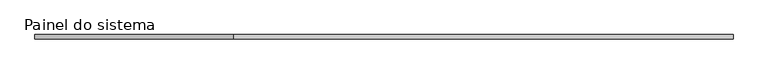
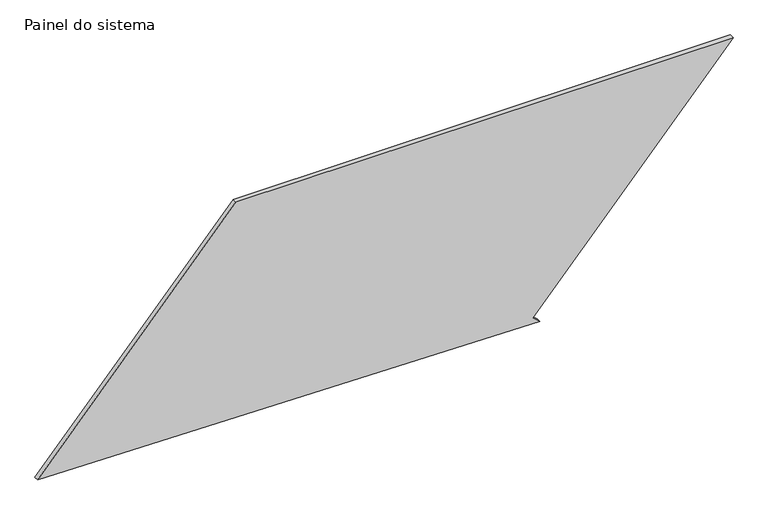
"""IFC4 building model written with IfcOpenShell, lengths in millimetres: plate geometry, Painel do sistema : Envidraçado."""

from ifc_helpers import new_model, si_unit, frame, origin, place, context, project, spatial, polyline, outline, extrude, source, transform, mapped, element, save


def painel_do_sistema_1ee32824(model_context):
    return source(origin(), model_context, "Body", "SweptSolid", [
        extrude(outline(polyline([(0.0, 853.2973256), (33.0713273, 815.7968281), (1287.5514622, 1922.1107677), (1287.5514622, -826.9931544), (45.767153, -1922.1107677), (0.0, 853.2973256)])), frame((0.0, 24.5, 0.0), z_axis=(0.0, 1.0, 0.0), x_axis=(0.0, 0.0, 1.0)), (0.0, 0.0, 1.0), 25.0),
    ])


if __name__ == "__main__":
    model = new_model("IFC4")
    model_context = context("Model", 3, world=origin())
    ifc_project = project(units=[si_unit("LENGTHUNIT", "METRE", prefix="MILLI")], contexts=[model_context])
    site = spatial("IfcSite", under=ifc_project)
    building = spatial("IfcBuilding", under=site)
    placement = place(None, origin())
    painel_do_sistema_shape = painel_do_sistema_1ee32824(model_context)
    element("IfcPlate", 1, ObjectType="Painel do sistema : Envidraçado", at=placement, inside=building, context=model_context, shape_type="MappedRepresentation", body=[
        mapped(painel_do_sistema_shape, transform((0.0, 0.0, 0.0), x_axis=(1.0, 0.0, 0.0), y_axis=(0.0, 1.0, 0.0), z_axis=(0.0, 0.0, 1.0))),
    ])
    save(model, "model.ifc")

# Revit data of these elements
# Type "Painel do sistema : Envidraçado"
#   Construction Type Id = "GSP4R"
#   Analytic Construction = "Vidraça única Pilkington 1/8 pol"
#   Visual Light Transmittance = 0.9
#   Solar Heat Gain Coefficient = 0.86
#   Heat Transfer Coefficient (U) = 6.7069 W/(m²·K)
# Element 1 (IfcPlate, "Painel do sistema : Envidraçado")
#   Materials on its faces: "Vidro"
# Materials
#   "Vidro": class "Vidro", colour RGB 0 128 192, transparency 0.9, Description = "Vidro de sílica", Cost = 0
